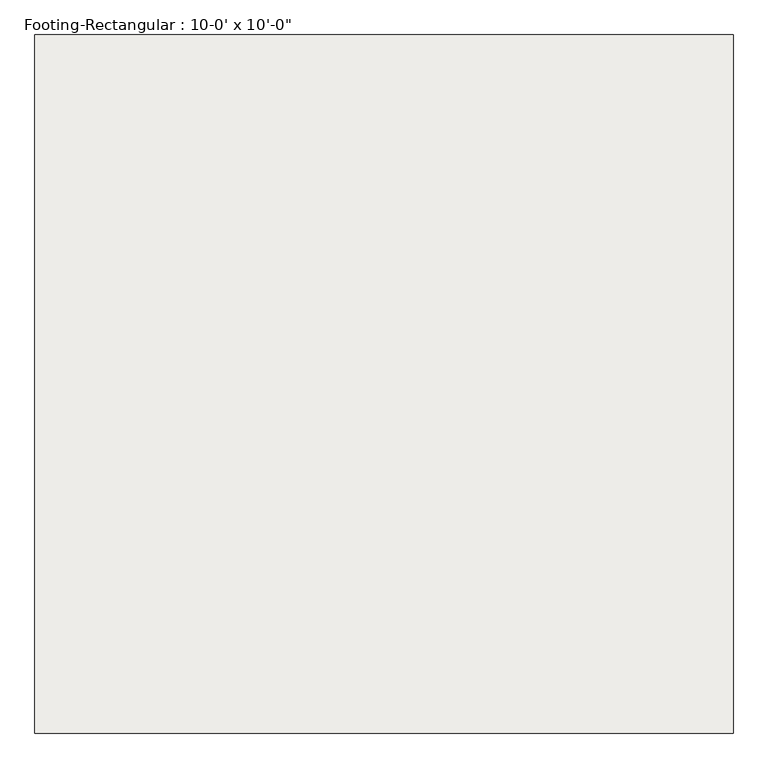
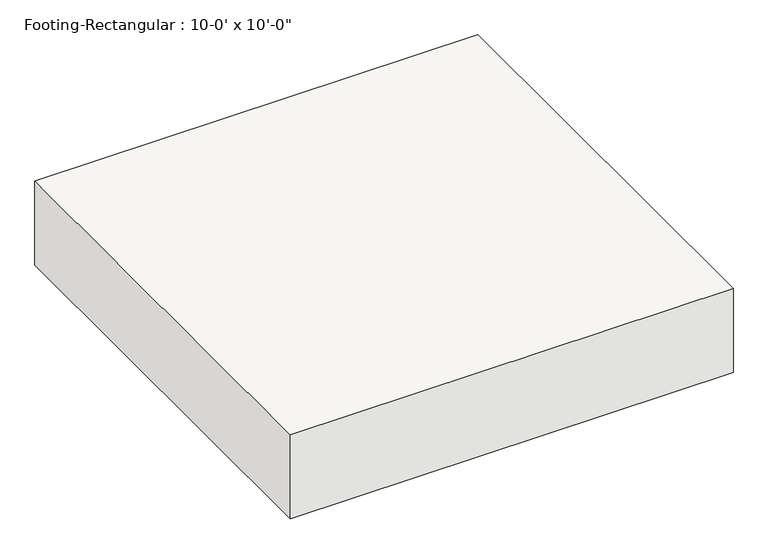
"""IFC4 building model written with IfcOpenShell, lengths in millimetres: slab geometry."""

from ifc_helpers import new_model, si_unit, frame, origin, place, context, project, spatial, polyline, outline, extrude, source, transform, mapped, element, save


def slab_5ce8dbd1(model_context):
    return source(origin(), model_context, "Body", "SweptSolid", [
        extrude(outline(polyline([(1524.0, 1524.0), (1524.0, -1524.0), (-1524.0, -1524.0), (-1524.0, 1524.0), (1524.0, 1524.0)])), frame((0.0, 0.0, -609.6), z_axis=(0.0, 0.0, 1.0), x_axis=(1.0, 0.0, 0.0)), (0.0, 0.0, 1.0), 609.6),
    ])


if __name__ == "__main__":
    model = new_model("IFC4")
    model_context = context("Model", 3, world=origin())
    ifc_project = project(units=[si_unit("LENGTHUNIT", "METRE", prefix="MILLI")], contexts=[model_context])
    site = spatial("IfcSite", under=ifc_project)
    building = spatial("IfcBuilding", under=site)
    placement = place(None, origin())
    slab_shape = slab_5ce8dbd1(model_context)
    element("IfcSlab", 1, ObjectType="Footing-Rectangular : 10-0' x 10'-0\"", at=placement, inside=building, context=model_context, shape_type="MappedRepresentation", body=[
        mapped(slab_shape, transform((0.0, 0.0, 0.0), x_axis=(1.0, 0.0, 0.0), y_axis=(0.0, 1.0, 0.0), z_axis=(0.0, 0.0, 1.0))),
    ])
    save(model, "model.ifc")

# Revit data of these elements
# Type "Footing-Rectangular : 10-0' x 10'-0\""
#   Assembly Code = "A1010100"
#   Width = 10' - 0"
#   Length = 10' - 0"
#   Thickness = 2' - 0"
#   Footing Material [instance default] = Concrete - Cast-in-Place Concrete
# Element 1 (IfcSlab, "Footing-Rectangular : 10-0' x 10'-0\"")
#   Materials on its faces: "Concrete - Cast-in-Place Concrete"
# Materials
#   "Concrete - Cast-in-Place Concrete": class "Concrete", colour RGB 192 192 192, transparency 0.4
